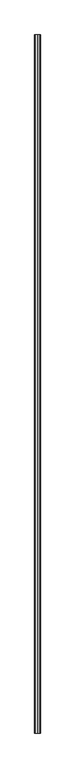
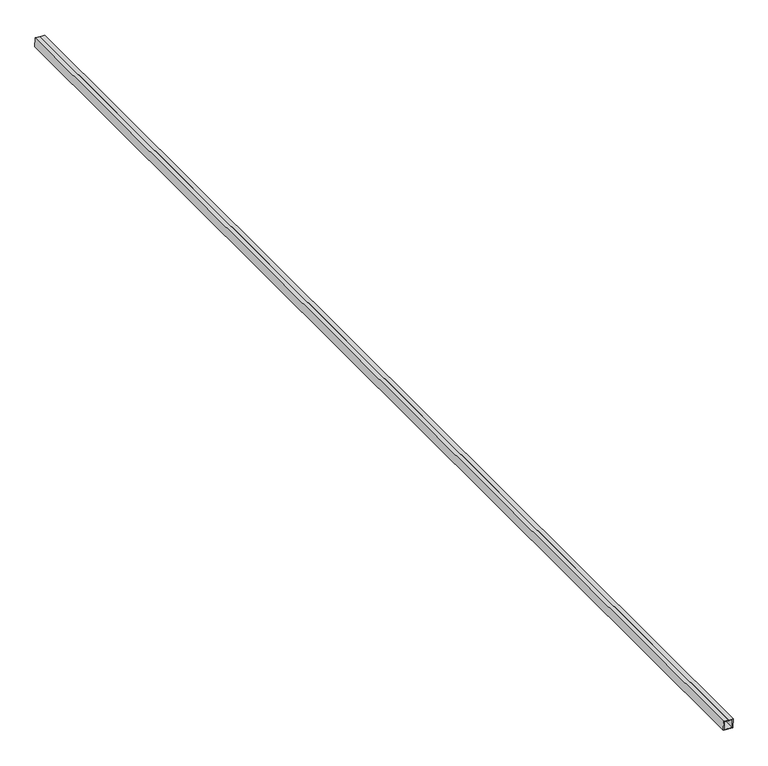
"""IFC4 building model written with IfcOpenShell, lengths in millimetres: proxy geometry, Inner panel:Inner panel:1:Inner panel:1 : Inner panel:Inner panel:300324:2:Inner panel:1:Inner panel:1 : Inner panel:Inner panel:300324:2 : Inner panel:Inner panel:1:Inner panel:1 : Inner panel:Inner panel:300324:300043:64 : Inner panel:Inner panel:1:Inner panel:1 : Inner panel:Inner panel:300324:2:Inner panel:1:Inner panel:1 : Inner panel:Inner panel:300324:2 : Inner panel:Inner panel:1:Inner panel:1 : Inner panel:Inner panel:300324:300043:308120."""

from ifc_helpers import new_model, si_unit, frame, origin, place, context, project, spatial, polyline, outline, extrude, source, transform, mapped, element, save


def generic_models_3ac9f363(model_context):
    return source(origin(), model_context, "Body", "SweptSolid", [
        extrude(outline(polyline([(3971.7309213, 802923.8565673), (3972.4909389, 802905.6161441), (3934.4239688, 802904.0300204), (3932.8378451, 802942.0969905), (3970.9048151, 802943.6831142), (3971.6648328, 802925.442691), (3969.2856471, 802925.3435583), (3968.6247622, 802941.2047958), (3935.3161634, 802939.8169376), (3936.7040217, 802906.5083387), (3970.0126205, 802907.896197), (3969.3517356, 802923.7574346), (3971.7309213, 802923.8565673)])), frame((0.0, -575657.4163839, 0.0), z_axis=(0.0, 1.0, 0.0), x_axis=(0.0, 0.0, 1.0)), (0.0, 0.0, 1.0), 4876.8),
    ])


if __name__ == "__main__":
    model = new_model("IFC4")
    model_context = context("Model", 3, world=origin())
    ifc_project = project(units=[si_unit("LENGTHUNIT", "METRE", prefix="MILLI")], contexts=[model_context])
    site = spatial("IfcSite", under=ifc_project)
    building = spatial("IfcBuilding", under=site)
    placement = place(None, origin())
    generic_models_shape = generic_models_3ac9f363(model_context)
    element("IfcBuildingElementProxy", 1, Name="Inner panel:Inner panel:1:Inner panel:1 : Inner panel:Inner panel:300324:2:Inner panel:1:Inner panel:1 : Inner panel:Inner panel:300324:2 : Inner panel:Inner panel:1:Inner panel:1 : Inner panel:Inner panel:300324:300043:64 : Inner panel:Inner panel:1:Inner panel:1 : Inner panel:Inner panel:300324:2:Inner panel:1:Inner panel:1 : Inner panel:Inner panel:300324:2 : Inner panel:Inner panel:1:Inner panel:1 : Inner panel:Inner panel:300324:300043:308120", ObjectType="Inner panel:Inner panel:1:Inner panel:1 : Inner panel:Inner panel:300324:2:Inner panel:1:Inner panel:1 : Inner panel:Inner panel:300324:2 : Inner panel:Inner panel:1:Inner panel:1 : Inner panel:Inner panel:300324:300043:64 : Inner panel:Inner panel:1:Inner panel:1 : Inner panel:Inner panel:300324:2:Inner panel:1:Inner panel:1 : Inner panel:Inner panel:300324:2 : Inner panel:Inner panel:1:Inner panel:1 : Inner panel:Inner panel:300324:300043:308120", at=placement, inside=building, context=model_context, shape_type="MappedRepresentation", body=[
        mapped(generic_models_shape, transform((0.0, 0.0, 0.0), x_axis=(1.0, 0.0, 0.0), y_axis=(0.0, 1.0, 0.0), z_axis=(0.0, 0.0, 1.0))),
    ])
    save(model, "model.ifc")

# Revit data of these elements
# Type "Inner panel:Inner panel:1:Inner panel:1 : Inner panel:Inner panel:300324:2:Inner panel:1:Inner panel:1 : Inner panel:Inner panel:300324:2 : Inner panel:Inner panel:1:Inner panel:1 : Inner panel:Inner panel:300324:300043:64 : Inner panel:Inner panel:1:Inner panel:1 : Inner panel:Inner panel:300324:2:Inner panel:1:Inner panel:1 : Inner panel:Inner panel:300324:2 : Inner panel:Inner panel:1:Inner panel:1 : Inner panel:Inner panel:300324:300043:308120"
#   NameOverride = "Inner panel:Inner panel:1:Inner panel:1 : Inner panel:Inner panel:300324:2:Inner panel:1:Inner panel:1 : Inner panel:Inner panel:300324:2 : Inner panel:Inner panel:1:Inner panel:1 : Inner panel:Inner panel:300324:300043:308120"
#   ObjectTypeOverride = "Inner panel:1:Inner panel:1 : Inner panel:Inner panel:300324:2 : Inner panel:Inner panel:1:Inner panel:1 : Inner panel:Inner panel:300324:300043"
#   Reference = "Inner panel"
#   Tag = "308120"
# Element 1 (IfcBuildingElementProxy, "Inner panel:Inner panel:1:Inner panel:1 : Inner panel:Inner panel:300324:2:Inner panel:1:Inner panel:1 : Inner panel:Inner panel:300324:2 : Inner panel:Inner panel:1:Inner panel:1 : Inner panel:Inner panel:300324:300043:64 : Inner panel:Inner panel:1:Inner panel:1 : Inner panel:Inner panel:300324:2:Inner panel:1:Inner panel:1 : Inner panel:Inner panel:300324:2 : Inner panel:Inner panel:1:Inner panel:1 : Inner panel:Inner panel:300324:300043:308120")
#   Materials on its faces: "1 1/2\" X 1 1/2\" SPLIT-SEAM SQUARE TUBING (~24\" CANTILEVER FROM C.L. OF GLULAM)"
# Materials
#   "1 1/2\" X 1 1/2\" SPLIT-SEAM SQUARE TUBING (~24\" CANTILEVER FROM C.L. OF GLULAM)": class "Unassigned", colour RGB 202 201 200, transparency 0, Cost = 0
